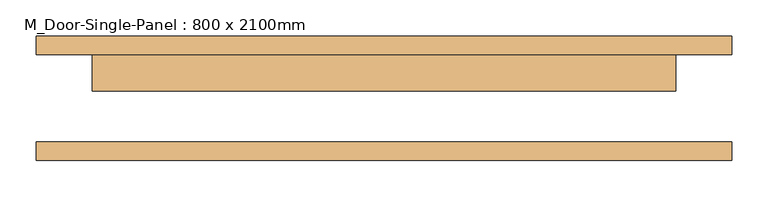
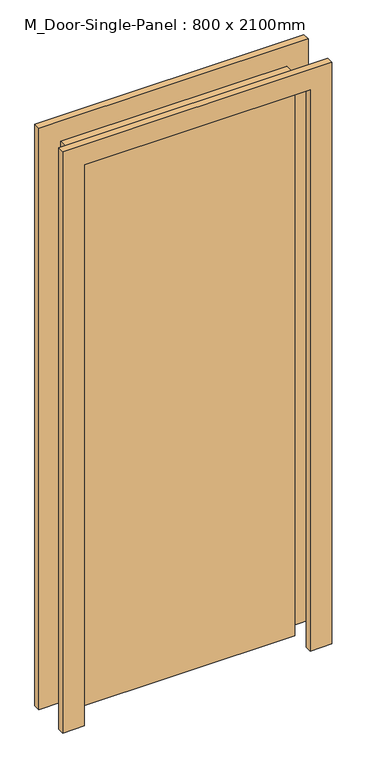
"""IFC4 building model written with IfcOpenShell, lengths in millimetres: door geometry, M_Door-Single-Panel : 800 x 2100mm."""

from ifc_helpers import new_model, si_unit, frame, origin, origin_with_axes, place, context, project, spatial, polyline, outline, extrude, source, transform, mapped, element, save


def m_door_single_panel_800_x_2100mm_7e59a417(model_context):
    return source(origin(), model_context, "Body", "SweptSolid", [
        extrude(outline(polyline([(400.0, 10.0), (-400.0, 10.0), (-400.0, 60.0), (400.0, 60.0), (400.0, 10.0)])), origin_with_axes(), (0.0, 0.0, 1.0), 2100.0),
        extrude(outline(polyline([(2176.2, -476.2), (0.0, -476.2), (0.0, -400.0), (2100.0, -400.0), (2100.0, 400.0), (0.0, 400.0), (0.0, 476.2), (2176.2, 476.2), (2176.2, -476.2)])), frame((0.0, 60.0, 0.0), z_axis=(0.0, 1.0, 0.0), x_axis=(0.0, 0.0, 1.0)), (0.0, 0.0, 1.0), 25.0),
        extrude(outline(polyline([(2176.2, 476.2), (2176.2, -476.2), (0.0, -476.2), (0.0, -400.0), (2100.0, -400.0), (2100.0, 400.0), (0.0, 400.0), (0.0, 476.2), (2176.2, 476.2)])), frame((0.0, -85.0, 0.0), z_axis=(0.0, 1.0, 0.0), x_axis=(0.0, 0.0, 1.0)), (0.0, 0.0, 1.0), 25.0),
    ])


if __name__ == "__main__":
    model = new_model("IFC4")
    model_context = context("Model", 3, world=origin())
    ifc_project = project(units=[si_unit("LENGTHUNIT", "METRE", prefix="MILLI")], contexts=[model_context])
    site = spatial("IfcSite", under=ifc_project)
    building = spatial("IfcBuilding", under=site)
    placement = place(None, origin())
    m_door_single_panel_800_x_2100mm_shape = m_door_single_panel_800_x_2100mm_7e59a417(model_context)
    element("IfcDoor", 1, ObjectType="M_Door-Single-Panel : 800 x 2100mm", at=placement, inside=building, context=model_context, shape_type="MappedRepresentation", body=[
        mapped(m_door_single_panel_800_x_2100mm_shape, transform((0.0, 0.0, 0.0), x_axis=(1.0, 0.0, 0.0), y_axis=(0.0, 1.0, 0.0), z_axis=(0.0, 0.0, 1.0))),
    ])
    save(model, "model.ifc")

# Revit data of these elements
# Type "M_Door-Single-Panel : 800 x 2100mm"
#   Type Mark = "41"
#   Construction Type Id = "DOOR"
#   Assembly Code = "C1020300"
#   Analytic Construction = "Wooden"
#   Thickness = 5 cm
#   Thermal Resistance (R) = 0.455703 (m²·K)/W
#   Swing Angle [instance default] = 90.00°
#   Heat Transfer Coefficient (U) = 2.19465 W/(m²·K)
#   Height = 210 cm
#   Trim Projection Ext = 2.5 cm
#   Trim Projection Int = 2.5 cm
#   Trim Width = 8 cm
#   Width = 80 cm
#   Panel Material = Wood - Birch - Solid Stained Light Low Gloss
#   Trim Material = Paint - Sienna
#   Visual Light Transmittance = 0
#   Solar Heat Gain Coefficient = 0
#   Function = (empty or 0)
#   Wall Closure = (empty or 0)
# Element 1 (IfcDoor, "M_Door-Single-Panel : 800 x 2100mm")
#   Materials on its faces: "Paint - Sienna", "Wood - Birch - Solid Stained Light Low Gloss"
# Materials
#   "Wood - Birch - Solid Stained Light Low Gloss": class "Wood", colour RGB 210 159 95, transparency 0, Cost = 0
#   "Paint - Sienna": class "Miscellaneous", colour RGB 118 70 51, transparency 0, Cost = 0
